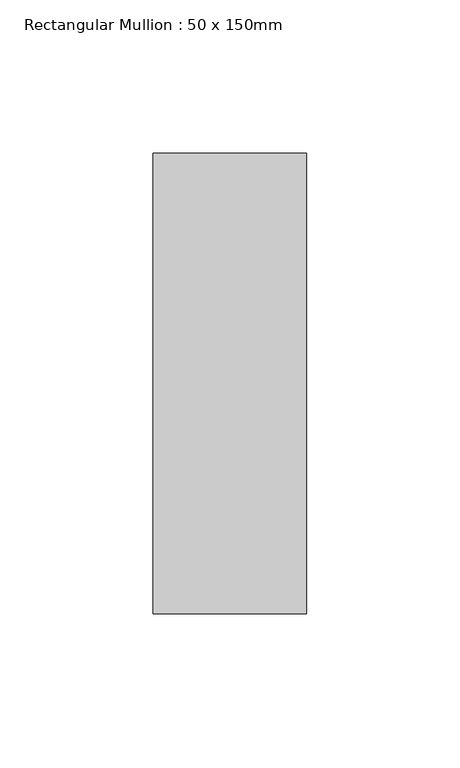
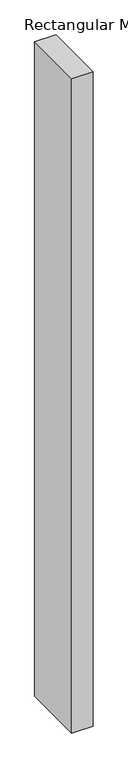
"""IFC4 building model written with IfcOpenShell, lengths in millimetres: member geometry, Rectangular Mullion : 50 x 150mm."""

import ifcopenshell
import ifcopenshell.guid

model = None  # the IFC model being written
_history = None  # IfcOwnerHistory: only IFC2X3 demands one
_inside = {}  # id of a spatial element -> (the spatial element, [elements in it])
_under = {}  # id of a project, library or spatial element -> (it, [spatial elements below it])
_declared = {}  # id of a project -> (the project, [libraries it declares])
_typed = {}  # id of a type object -> (the type object, [elements of that type])
_made_of = {}  # id of a material, layer set ... -> (it, [elements and type objects made of it])


def new_model(schema):
    """Start an empty IFC model of exactly this schema.

    Asked for "IFC4X3", IfcOpenShell would pick the latest addendum, in which some entities
    have other attributes; the version numbers below select the first issue.
    IFC2X3 requires an IfcOwnerHistory on every rooted entity: one is made here for all.
    """
    global model, _history
    if schema == "IFC4X3":
        model = ifcopenshell.file(schema_version=(4, 3, 0, 0))
    else:
        model = ifcopenshell.file(schema=schema)
    _inside.clear()
    _under.clear()
    _declared.clear()
    _typed.clear()
    _made_of.clear()
    _history = None
    if model.schema == "IFC2X3":
        org = make("IfcOrganization", Name="unknown")
        user = make(
            "IfcPersonAndOrganization",
            ThePerson=make("IfcPerson", FamilyName="unknown"),
            TheOrganization=org,
        )
        app = make(
            "IfcApplication",
            ApplicationDeveloper=org,
            Version="unknown",
            ApplicationFullName="unknown",
            ApplicationIdentifier="unknown",
        )
        _history = make(
            "IfcOwnerHistory",
            OwningUser=user,
            OwningApplication=app,
            ChangeAction="ADDED",
            CreationDate=0,
        )
    return model


def make(cls, **values):
    """One entity of the class cls with the attributes given. An attribute that is None is left unset."""
    return model.create_entity(
        cls, **{name: value for name, value in values.items() if value is not None}
    )


def rooted(cls, **values):
    """An entity with a GlobalId (a new one), such as an element, a storey or a relation."""
    return make(cls, GlobalId=ifcopenshell.guid.new(), OwnerHistory=_history, **values)


def si_unit(unit_type, name, prefix=None):
    """IfcSIUnit, for example si_unit("LENGTHUNIT", "METRE", prefix="MILLI")."""
    return make("IfcSIUnit", UnitType=unit_type, Prefix=prefix, Name=name)


def assignment(units):
    """IfcUnitAssignment: the units of a project."""
    return None if units is None else make("IfcUnitAssignment", Units=units)


def point(xyz):
    """IfcCartesianPoint."""
    return None if xyz is None else make("IfcCartesianPoint", Coordinates=xyz)


def direction(xyz):
    """IfcDirection."""
    return None if xyz is None else make("IfcDirection", DirectionRatios=xyz)


def frame(location, z_axis=None, x_axis=None):
    """IfcAxis2Placement3D, a coordinate frame: its origin and axes. An axis left out is left unset."""
    return make(
        "IfcAxis2Placement3D",
        Location=point(location),
        Axis=direction(z_axis),
        RefDirection=direction(x_axis),
    )


def origin():
    """The frame at (0, 0, 0) with its axes left unset."""
    return frame((0.0, 0.0, 0.0))


def place(relative_to, where):
    """IfcLocalPlacement: puts the frame where relative to a parent placement (None: the world)."""
    return make(
        "IfcLocalPlacement", PlacementRelTo=relative_to, RelativePlacement=where
    )


def context(
    kind, dimensions, precision=None, world=None, true_north=None, identifier=None
):
    """IfcGeometricRepresentationContext, for example the 3D "Model" context."""
    return make(
        "IfcGeometricRepresentationContext",
        ContextIdentifier=identifier,
        ContextType=kind,
        CoordinateSpaceDimension=dimensions,
        Precision=precision,
        WorldCoordinateSystem=world,
        TrueNorth=true_north,
    )


def project(units=None, contexts=None):
    """IfcProject with its units and contexts."""
    return rooted(
        "IfcProject",
        Name="project",
        RepresentationContexts=contexts,
        UnitsInContext=assignment(units),
    )


def spatial(cls, under=None, at=None, **own):
    """A site, building, storey or space (cls), placed at a placement, below another one or the project."""
    s = rooted(cls, ObjectPlacement=at, **own)
    if under is not None:
        _under.setdefault(under.id(), (under, []))[1].append(s)
    return s


def polyline(points):
    """IfcPolyline through the points."""
    return make("IfcPolyline", Points=[point(p) for p in points])


def outline(outer, holes=None, kind="AREA"):
    """IfcArbitraryClosedProfileDef: a profile drawn as a closed curve; with holes, ...WithVoids."""
    if holes is None:
        return make("IfcArbitraryClosedProfileDef", ProfileType=kind, OuterCurve=outer)
    return make(
        "IfcArbitraryProfileDefWithVoids",
        ProfileType=kind,
        OuterCurve=outer,
        InnerCurves=holes,
    )


def extrude(swept, where, along, depth):
    """IfcExtrudedAreaSolid: the profile swept, set in the frame where, extruded along a direction by depth."""
    return make(
        "IfcExtrudedAreaSolid",
        SweptArea=swept,
        Position=where,
        ExtrudedDirection=direction(along),
        Depth=depth,
    )


def shape(context_of_items, identifier, shape_type, items):
    """IfcShapeRepresentation: the items that make up one representation, for example the "Body"."""
    return make(
        "IfcShapeRepresentation",
        ContextOfItems=context_of_items,
        RepresentationIdentifier=identifier,
        RepresentationType=shape_type,
        Items=items,
    )


def source(mapping_origin, context_of_items, identifier, shape_type, items):
    """IfcRepresentationMap: a shape defined once, which mapped items show again and again."""
    return make(
        "IfcRepresentationMap",
        MappingOrigin=mapping_origin,
        MappedRepresentation=shape(context_of_items, identifier, shape_type, items),
    )


def transform(
    local_origin,
    x_axis=None,
    y_axis=None,
    z_axis=None,
    scale=None,
    scale2=None,
    scale3=None,
    uniform=True,
):
    """IfcCartesianTransformationOperator3D, or its non-uniform kind. x_axis, y_axis, z_axis: its Axis1, 2, 3."""
    if uniform:
        return make(
            "IfcCartesianTransformationOperator3D",
            Axis1=direction(x_axis),
            Axis2=direction(y_axis),
            LocalOrigin=point(local_origin),
            Scale=scale,
            Axis3=direction(z_axis),
        )
    return make(
        "IfcCartesianTransformationOperator3DnonUniform",
        Axis1=direction(x_axis),
        Axis2=direction(y_axis),
        LocalOrigin=point(local_origin),
        Scale=scale,
        Axis3=direction(z_axis),
        Scale2=scale2,
        Scale3=scale3,
    )


def mapped(mapping_source, mapping_target):
    """IfcMappedItem: shows the shape of a source again, moved by a transform."""
    return make(
        "IfcMappedItem", MappingSource=mapping_source, MappingTarget=mapping_target
    )


def made_of(thing, what):
    """Note that an element or type object is made of a material, layer set ...; save() writes the relation."""
    if what is not None:
        _made_of.setdefault(what.id(), (what, []))[1].append(thing)
    return thing


def element(
    cls,
    number,
    at=None,
    inside=None,
    cuts=None,
    type_object=None,
    material=None,
    context=None,
    identifier="Body",
    shape_type=None,
    held_by="IfcProductDefinitionShape",
    body=None,
    shapes=None,
    **own,
):
    """One element of the class cls, such as IfcWall. Its Tag is "e" and its number.

    at: its placement. inside: the storey or other place that contains it. cuts: it is an
    opening in that element (IfcRelVoidsElement). A single representation is given by context,
    identifier, shape_type and body (its items); several are given by shapes. held_by: the class
    of the entity that holds the representations. save() writes the other relations.
    """
    e = rooted(cls, Tag="e%d" % number, ObjectPlacement=at, **own)
    if body is not None:
        shapes = [shape(context, identifier, shape_type, body)]
    if shapes is not None:
        e.Representation = make(held_by, Representations=shapes)
    if inside is not None:
        _inside.setdefault(inside.id(), (inside, []))[1].append(e)
    if cuts is not None:
        rooted(
            "IfcRelVoidsElement", RelatingBuildingElement=cuts, RelatedOpeningElement=e
        )
    if type_object is not None:
        _typed.setdefault(type_object.id(), (type_object, []))[1].append(e)
    return made_of(e, material)


def aggregate(whole, parts):
    """IfcRelAggregates: a whole, such as a stair, and the parts it consists of."""
    return rooted("IfcRelAggregates", RelatingObject=whole, RelatedObjects=parts)


def save(model, path):
    """Write the relations noted so far, then the file.

    IfcRelAggregates (storeys below a building ...), IfcRelContainedInSpatialStructure (elements
    in a storey), IfcRelDefinesByType, IfcRelAssociatesMaterial and IfcRelDeclares: one each for
    every whole, place, type object, material and project.
    """
    for whole, parts in _under.values():
        aggregate(whole, parts)
    for where, things in _inside.values():
        rooted(
            "IfcRelContainedInSpatialStructure",
            RelatedElements=things,
            RelatingStructure=where,
        )
    for kind, things in _typed.values():
        rooted("IfcRelDefinesByType", RelatedObjects=things, RelatingType=kind)
    for what, things in _made_of.values():
        rooted("IfcRelAssociatesMaterial", RelatedObjects=things, RelatingMaterial=what)
    for by, libraries in _declared.values():
        rooted("IfcRelDeclares", RelatingContext=by, RelatedDefinitions=libraries)
    model.write(path)


def rectangular_mullion_50_x_150mm_f3f87aca(model_context):
    return source(origin(), model_context, "Body", "SweptSolid", [
        extrude(outline(polyline([(0.0, 75.0), (0.0, -75.0), (-50.0, -75.0), (-50.0, 75.0), (0.0, 75.0)])), frame((0.0, 0.0, -1620.0), z_axis=(0.0, 0.0, 1.0), x_axis=(1.0, 0.0, 0.0)), (0.0, 0.0, 1.0), 1620.0),
    ])


if __name__ == "__main__":
    model = new_model("IFC4")
    model_context = context("Model", 3, world=origin())
    ifc_project = project(units=[si_unit("LENGTHUNIT", "METRE", prefix="MILLI")], contexts=[model_context])
    site = spatial("IfcSite", under=ifc_project)
    building = spatial("IfcBuilding", under=site)
    placement = place(None, origin())
    rectangular_mullion_50_x_150mm_shape = rectangular_mullion_50_x_150mm_f3f87aca(model_context)
    element("IfcMember", 1, ObjectType="Rectangular Mullion : 50 x 150mm", at=placement, inside=building, context=model_context, shape_type="MappedRepresentation", body=[
        mapped(rectangular_mullion_50_x_150mm_shape, transform((0.0, 0.0, 0.0), x_axis=(1.0, 0.0, 0.0), y_axis=(0.0, 1.0, 0.0), z_axis=(0.0, 0.0, 1.0))),
    ])
    save(model, "model.ifc")

# Revit data of these elements
# Type "Rectangular Mullion : 50 x 150mm"
#   built-in parameter 1007304 = 0.492126 (stored number, unit not read)
#   built-in parameter 1007301 = 0.082021 (stored number, unit not read)
#   built-in parameter 1007300 = 0.082021 (stored number, unit not read)
# Element 1 (IfcMember, "Rectangular Mullion : 50 x 150mm")
#   Materials on its faces: "Metal - Aluminium"
# Materials
#   "Metal - Aluminium": class "Metal", colour RGB 247 247 247, transparency 0
